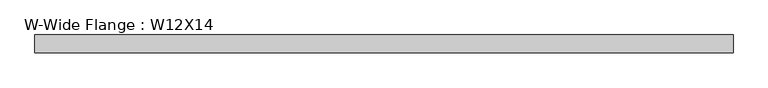
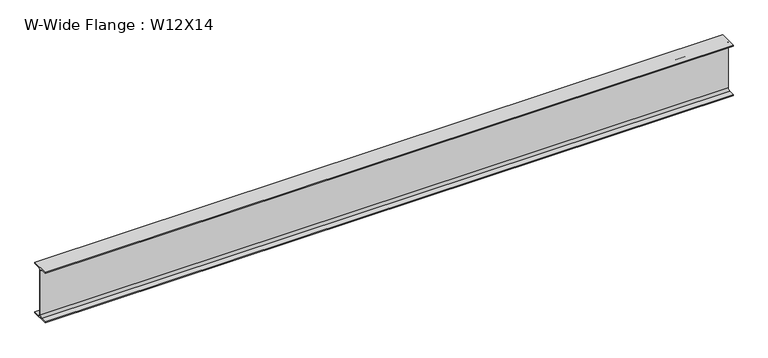
"""IFC4 building model written with IfcOpenShell, lengths in millimetres: beam geometry, W-Wide Flange : W12X14."""

from ifc_helpers import new_model, si_unit, point, frame, frame_2d, origin, place, context, project, spatial, polyline, circle_curve, trimmed, segment, composite_curve, outline, extrude, source, transform, mapped, element, save


def w_wide_flange_w12x14_35562f8b(model_context):
    return source(origin(), model_context, "Body", "SweptSolid", [
        extrude(outline(composite_curve([segment(polyline([(50.419, -145.415), (50.419, -151.13), (-50.419, -151.13), (-50.419, -145.415), (-15.875, -145.415)]), True, "CONTINUOUS"), segment(trimmed(circle_curve(frame_2d((-15.875, -132.08)), 13.335), [point((-15.875, -145.415))], [point((-2.54, -132.08))], True, "CARTESIAN"), True, "CONTINUOUS"), segment(polyline([(-2.54, -132.08), (-2.54, 132.08)]), True, "CONTINUOUS"), segment(trimmed(circle_curve(frame_2d((-15.875, 132.08)), 13.335), [point((-2.54, 132.08))], [point((-15.875, 145.415))], True, "CARTESIAN"), True, "CONTINUOUS"), segment(polyline([(-15.875, 145.415), (-50.419, 145.415), (-50.419, 151.13), (50.419, 151.13), (50.419, 145.415), (15.875, 145.415)]), True, "CONTINUOUS"), segment(trimmed(circle_curve(frame_2d((15.875, 132.08)), 13.335), [point((15.875, 145.415))], [point((2.54, 132.08))], True, "CARTESIAN"), True, "CONTINUOUS"), segment(polyline([(2.54, 132.08), (2.54, -132.08)]), True, "CONTINUOUS"), segment(trimmed(circle_curve(frame_2d((15.875, -132.08)), 13.335), [point((2.54, -132.08))], [point((15.875, -145.415))], True, "CARTESIAN"), True, "CONTINUOUS"), segment(polyline([(15.875, -145.415), (50.419, -145.415)]), True, "CONTINUOUS")], self_intersect=False)), frame((-1943.1, 0.0, 0.0), z_axis=(1.0, 0.0, 0.0), x_axis=(0.0, 1.0, 0.0)), (0.0, 0.0, 1.0), 3898.773),
    ])


if __name__ == "__main__":
    model = new_model("IFC4")
    model_context = context("Model", 3, world=origin())
    ifc_project = project(units=[si_unit("LENGTHUNIT", "METRE", prefix="MILLI")], contexts=[model_context])
    site = spatial("IfcSite", under=ifc_project)
    building = spatial("IfcBuilding", under=site)
    placement = place(None, origin())
    w_wide_flange_w12x14_shape = w_wide_flange_w12x14_35562f8b(model_context)
    element("IfcBeam", 1, ObjectType="W-Wide Flange : W12X14", at=placement, inside=building, context=model_context, shape_type="MappedRepresentation", body=[
        mapped(w_wide_flange_w12x14_shape, transform((0.0, 0.0, 0.0), x_axis=(1.0, 0.0, 0.0), y_axis=(0.0, 1.0, 0.0), z_axis=(0.0, 0.0, 1.0))),
    ])
    save(model, "model.ifc")

# Revit data of these elements
# Type "W-Wide Flange : W12X14"
#   Assembly Code = "B10"
#   W = 14
#   Length [instance default] = 5' - 0"
#   bf = 0' - 3.97"
#   d = 0' - 11.9"
#   k = 0' - 0 3/4"
#   k2 = 0' - 0.525"
#   tf = 0' - 0.225"
#   tw = 0' - 0.2"
#   A = 0.0288889 SF
#   Structural Material [instance default] = Steel ASTM A992
# Element 1 (IfcBeam, "W-Wide Flange : W12X14")
#   Materials on its faces: "Steel ASTM A992"
# Materials
#   "Steel ASTM A992": class "Metal", colour RGB 199 199 199, transparency 0, Description = "Structural steel 50ksi", Cost = 0
